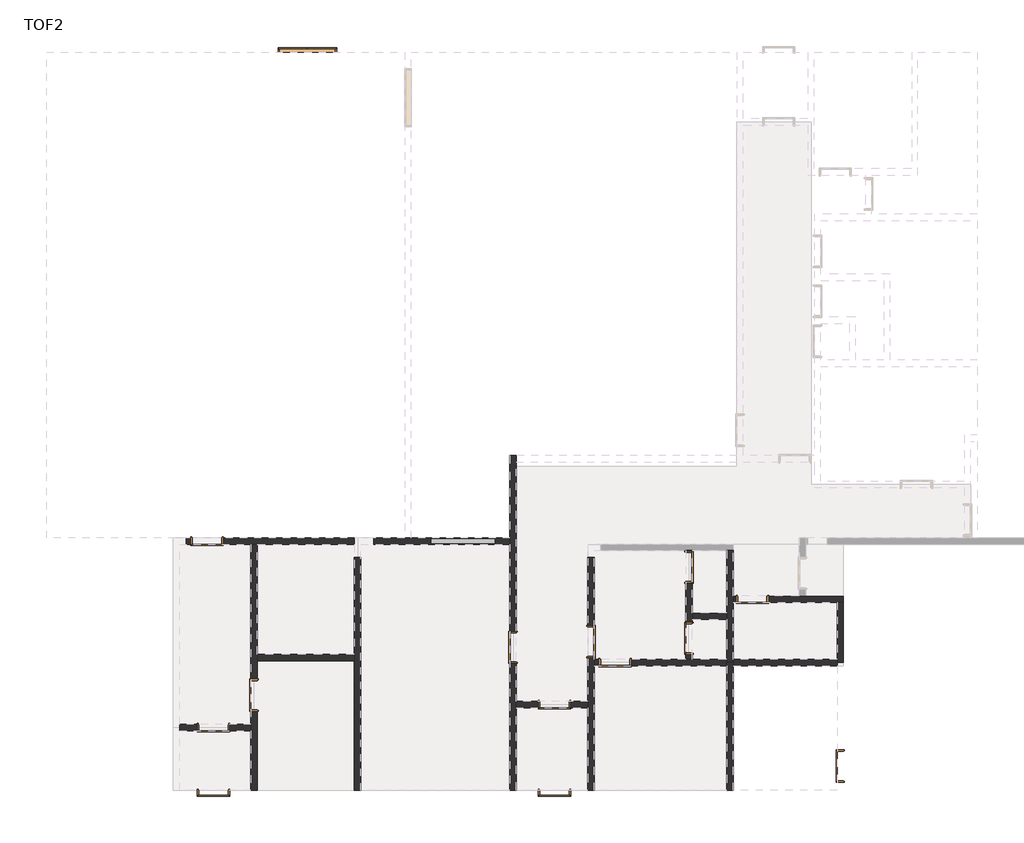
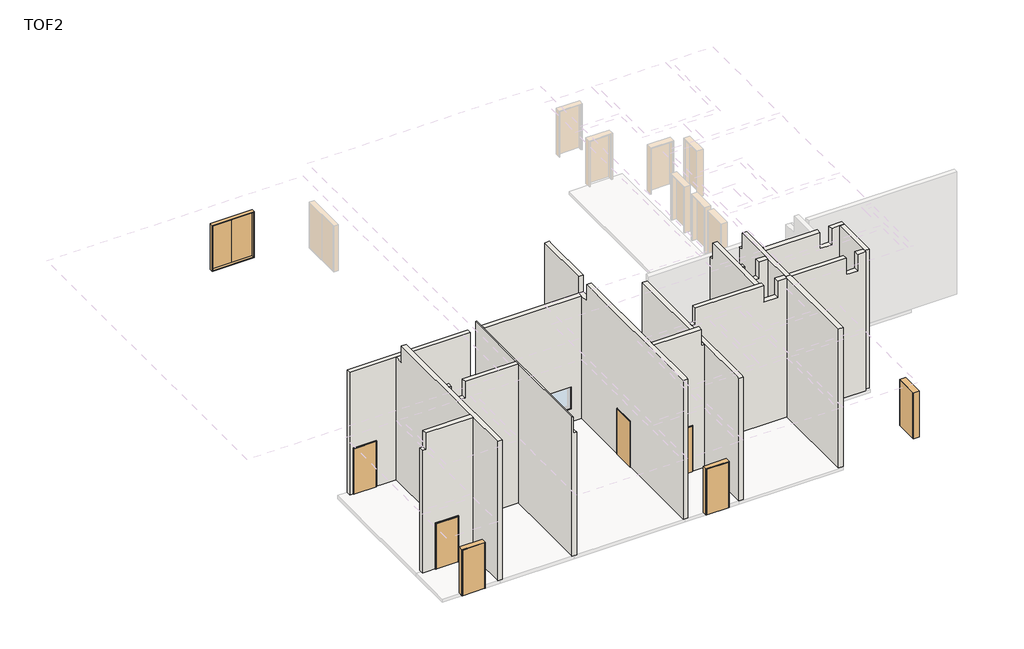
# One storey, part 1 of 2: 16 walls, 14 doors.
"""IFC4 building model written with IfcOpenShell, lengths in millimetres."""

import ifcopenshell
import ifcopenshell.guid

model = None  # the IFC model being written
_history = None  # IfcOwnerHistory: only IFC2X3 demands one
_inside = {}  # id of a spatial element -> (the spatial element, [elements in it])
_under = {}  # id of a project, library or spatial element -> (it, [spatial elements below it])
_declared = {}  # id of a project -> (the project, [libraries it declares])
_typed = {}  # id of a type object -> (the type object, [elements of that type])
_made_of = {}  # id of a material, layer set ... -> (it, [elements and type objects made of it])


def new_model(schema):
    """Start an empty IFC model of exactly this schema.

    Asked for "IFC4X3", IfcOpenShell would pick the latest addendum, in which some entities
    have other attributes; the version numbers below select the first issue.
    IFC2X3 requires an IfcOwnerHistory on every rooted entity: one is made here for all.
    """
    global model, _history
    if schema == "IFC4X3":
        model = ifcopenshell.file(schema_version=(4, 3, 0, 0))
    else:
        model = ifcopenshell.file(schema=schema)
    _inside.clear()
    _under.clear()
    _declared.clear()
    _typed.clear()
    _made_of.clear()
    _history = None
    if model.schema == "IFC2X3":
        org = make("IfcOrganization", Name="unknown")
        user = make(
            "IfcPersonAndOrganization",
            ThePerson=make("IfcPerson", FamilyName="unknown"),
            TheOrganization=org,
        )
        app = make(
            "IfcApplication",
            ApplicationDeveloper=org,
            Version="unknown",
            ApplicationFullName="unknown",
            ApplicationIdentifier="unknown",
        )
        _history = make(
            "IfcOwnerHistory",
            OwningUser=user,
            OwningApplication=app,
            ChangeAction="ADDED",
            CreationDate=0,
        )
    return model


def make(cls, **values):
    """One entity of the class cls with the attributes given. An attribute that is None is left unset."""
    return model.create_entity(
        cls, **{name: value for name, value in values.items() if value is not None}
    )


def rooted(cls, **values):
    """An entity with a GlobalId (a new one), such as an element, a storey or a relation."""
    return make(cls, GlobalId=ifcopenshell.guid.new(), OwnerHistory=_history, **values)


def si_unit(unit_type, name, prefix=None):
    """IfcSIUnit, for example si_unit("LENGTHUNIT", "METRE", prefix="MILLI")."""
    return make("IfcSIUnit", UnitType=unit_type, Prefix=prefix, Name=name)


def assignment(units):
    """IfcUnitAssignment: the units of a project."""
    return None if units is None else make("IfcUnitAssignment", Units=units)


def point(xyz):
    """IfcCartesianPoint."""
    return None if xyz is None else make("IfcCartesianPoint", Coordinates=xyz)


def direction(xyz):
    """IfcDirection."""
    return None if xyz is None else make("IfcDirection", DirectionRatios=xyz)


def frame(location, z_axis=None, x_axis=None):
    """IfcAxis2Placement3D, a coordinate frame: its origin and axes. An axis left out is left unset."""
    return make(
        "IfcAxis2Placement3D",
        Location=point(location),
        Axis=direction(z_axis),
        RefDirection=direction(x_axis),
    )


def origin():
    """The frame at (0, 0, 0) with its axes left unset."""
    return frame((0.0, 0.0, 0.0))


def origin_with_axes():
    """The frame at (0, 0, 0) with the z axis (0, 0, 1) and the x axis (1, 0, 0) written out."""
    return frame((0.0, 0.0, 0.0), z_axis=(0.0, 0.0, 1.0), x_axis=(1.0, 0.0, 0.0))


def place(relative_to, where):
    """IfcLocalPlacement: puts the frame where relative to a parent placement (None: the world)."""
    return make(
        "IfcLocalPlacement", PlacementRelTo=relative_to, RelativePlacement=where
    )


def context(
    kind, dimensions, precision=None, world=None, true_north=None, identifier=None
):
    """IfcGeometricRepresentationContext, for example the 3D "Model" context."""
    return make(
        "IfcGeometricRepresentationContext",
        ContextIdentifier=identifier,
        ContextType=kind,
        CoordinateSpaceDimension=dimensions,
        Precision=precision,
        WorldCoordinateSystem=world,
        TrueNorth=true_north,
    )


def project(units=None, contexts=None):
    """IfcProject with its units and contexts."""
    return rooted(
        "IfcProject",
        Name="project",
        RepresentationContexts=contexts,
        UnitsInContext=assignment(units),
    )


def spatial(cls, under=None, at=None, **own):
    """A site, building, storey or space (cls), placed at a placement, below another one or the project."""
    s = rooted(cls, ObjectPlacement=at, **own)
    if under is not None:
        _under.setdefault(under.id(), (under, []))[1].append(s)
    return s


def polyline(points):
    """IfcPolyline through the points."""
    return make("IfcPolyline", Points=[point(p) for p in points])


def outline(outer, holes=None, kind="AREA"):
    """IfcArbitraryClosedProfileDef: a profile drawn as a closed curve; with holes, ...WithVoids."""
    if holes is None:
        return make("IfcArbitraryClosedProfileDef", ProfileType=kind, OuterCurve=outer)
    return make(
        "IfcArbitraryProfileDefWithVoids",
        ProfileType=kind,
        OuterCurve=outer,
        InnerCurves=holes,
    )


def extrude(swept, where, along, depth):
    """IfcExtrudedAreaSolid: the profile swept, set in the frame where, extruded along a direction by depth."""
    return make(
        "IfcExtrudedAreaSolid",
        SweptArea=swept,
        Position=where,
        ExtrudedDirection=direction(along),
        Depth=depth,
    )


def faces_of(points, faces, orient=None, outer=None):
    """IfcFace entities. A face is a list of loops; a loop is a list of indices into points, from 0.

    orient and outer hold one flag for each loop. By default every Orientation is true, the
    first loop of a face is its IfcFaceOuterBound and the others are IfcFaceBound.
    """
    made = []
    for i, loops in enumerate(faces):
        bounds = []
        for j, loop in enumerate(loops):
            is_outer = j == 0 if outer is None else outer[i][j]
            bounds.append(
                make(
                    "IfcFaceOuterBound" if is_outer else "IfcFaceBound",
                    Bound=make("IfcPolyLoop", Polygon=[points[k] for k in loop]),
                    Orientation=True if orient is None else orient[i][j],
                )
            )
        made.append(make("IfcFace", Bounds=bounds))
    return made


def faceted_brep(points, faces, orient=None, outer=None, voids=None):
    """IfcFacetedBrep: a solid bounded by flat faces; with voids (closed shells), ...WithVoids."""
    shared = [point(p) for p in points]
    hull = make("IfcClosedShell", CfsFaces=faces_of(shared, faces, orient, outer))
    if voids is None:
        return make("IfcFacetedBrep", Outer=hull)
    return make(
        "IfcFacetedBrepWithVoids",
        Outer=hull,
        Voids=[
            make(cls, CfsFaces=faces_of(shared, fs, o, b)) for cls, fs, o, b in voids
        ],
    )


def shape(context_of_items, identifier, shape_type, items):
    """IfcShapeRepresentation: the items that make up one representation, for example the "Body"."""
    return make(
        "IfcShapeRepresentation",
        ContextOfItems=context_of_items,
        RepresentationIdentifier=identifier,
        RepresentationType=shape_type,
        Items=items,
    )


def source(mapping_origin, context_of_items, identifier, shape_type, items):
    """IfcRepresentationMap: a shape defined once, which mapped items show again and again."""
    return make(
        "IfcRepresentationMap",
        MappingOrigin=mapping_origin,
        MappedRepresentation=shape(context_of_items, identifier, shape_type, items),
    )


def transform(
    local_origin,
    x_axis=None,
    y_axis=None,
    z_axis=None,
    scale=None,
    scale2=None,
    scale3=None,
    uniform=True,
):
    """IfcCartesianTransformationOperator3D, or its non-uniform kind. x_axis, y_axis, z_axis: its Axis1, 2, 3."""
    if uniform:
        return make(
            "IfcCartesianTransformationOperator3D",
            Axis1=direction(x_axis),
            Axis2=direction(y_axis),
            LocalOrigin=point(local_origin),
            Scale=scale,
            Axis3=direction(z_axis),
        )
    return make(
        "IfcCartesianTransformationOperator3DnonUniform",
        Axis1=direction(x_axis),
        Axis2=direction(y_axis),
        LocalOrigin=point(local_origin),
        Scale=scale,
        Axis3=direction(z_axis),
        Scale2=scale2,
        Scale3=scale3,
    )


def mapped(mapping_source, mapping_target):
    """IfcMappedItem: shows the shape of a source again, moved by a transform."""
    return make(
        "IfcMappedItem", MappingSource=mapping_source, MappingTarget=mapping_target
    )


def made_of(thing, what):
    """Note that an element or type object is made of a material, layer set ...; save() writes the relation."""
    if what is not None:
        _made_of.setdefault(what.id(), (what, []))[1].append(thing)
    return thing


def element(
    cls,
    number,
    at=None,
    inside=None,
    cuts=None,
    type_object=None,
    material=None,
    context=None,
    identifier="Body",
    shape_type=None,
    held_by="IfcProductDefinitionShape",
    body=None,
    shapes=None,
    **own,
):
    """One element of the class cls, such as IfcWall. Its Tag is "e" and its number.

    at: its placement. inside: the storey or other place that contains it. cuts: it is an
    opening in that element (IfcRelVoidsElement). A single representation is given by context,
    identifier, shape_type and body (its items); several are given by shapes. held_by: the class
    of the entity that holds the representations. save() writes the other relations.
    """
    e = rooted(cls, Tag="e%d" % number, ObjectPlacement=at, **own)
    if body is not None:
        shapes = [shape(context, identifier, shape_type, body)]
    if shapes is not None:
        e.Representation = make(held_by, Representations=shapes)
    if inside is not None:
        _inside.setdefault(inside.id(), (inside, []))[1].append(e)
    if cuts is not None:
        rooted(
            "IfcRelVoidsElement", RelatingBuildingElement=cuts, RelatedOpeningElement=e
        )
    if type_object is not None:
        _typed.setdefault(type_object.id(), (type_object, []))[1].append(e)
    return made_of(e, material)


def aggregate(whole, parts):
    """IfcRelAggregates: a whole, such as a stair, and the parts it consists of."""
    return rooted("IfcRelAggregates", RelatingObject=whole, RelatedObjects=parts)


def save(model, path):
    """Write the relations noted so far, then the file.

    IfcRelAggregates (storeys below a building ...), IfcRelContainedInSpatialStructure (elements
    in a storey), IfcRelDefinesByType, IfcRelAssociatesMaterial and IfcRelDeclares: one each for
    every whole, place, type object, material and project.
    """
    for whole, parts in _under.values():
        aggregate(whole, parts)
    for where, things in _inside.values():
        rooted(
            "IfcRelContainedInSpatialStructure",
            RelatedElements=things,
            RelatingStructure=where,
        )
    for kind, things in _typed.values():
        rooted("IfcRelDefinesByType", RelatedObjects=things, RelatingType=kind)
    for what, things in _made_of.values():
        rooted("IfcRelAssociatesMaterial", RelatedObjects=things, RelatingMaterial=what)
    for by, libraries in _declared.values():
        rooted("IfcRelDeclares", RelatingContext=by, RelatedDefinitions=libraries)
    model.write(path)


def double_door_steel_580823b0(model_context):
    return source(origin(), model_context, "Body", "SolidModel", [
        extrude(outline(polyline([(880.0, 35.0), (0.0, 35.0), (0.0, 75.0), (880.0, 75.0), (880.0, 35.0)])), frame((0.0, 0.0, 20.0), z_axis=(0.0, 0.0, 1.0), x_axis=(1.0, 0.0, 0.0)), (0.0, 0.0, 1.0), 2060.0),
        extrude(outline(polyline([(0.0, 35.0), (-880.0, 35.0), (-880.0, 75.0), (0.0, 75.0), (0.0, 35.0)])), frame((0.0, 0.0, 20.0), z_axis=(0.0, 0.0, 1.0), x_axis=(1.0, 0.0, 0.0)), (0.0, 0.0, 1.0), 2060.0),
        faceted_brep([(900.0, -75.0, 2100.0), (900.0, 75.0, 2100.0), (-900.0, 75.0, 2100.0), (-900.0, -75.0, 2100.0), (865.0, 35.0, 2065.0), (865.0, -75.0, 2065.0), (-865.0, -75.0, 2065.0), (-865.0, 35.0, 2065.0), (880.0, 75.0, 2080.0), (880.0, 35.0, 2080.0), (-880.0, 35.0, 2080.0), (-880.0, 75.0, 2080.0), (-900.0, 75.0, 0.0), (-900.0, -75.0, 0.0), (-865.0, -75.0, 35.0), (-865.0, 35.0, 35.0), (-880.0, 35.0, 20.0), (-880.0, 75.0, 20.0), (900.0, 75.0, 0.0), (880.0, 75.0, 20.0), (900.0, -75.0, 0.0), (865.0, -75.0, 35.0), (865.0, 35.0, 35.0), (880.0, 35.0, 20.0)], [[[0, 1, 2, 3]], [[4, 5, 6, 7]], [[8, 9, 10, 11]], [[3, 2, 12, 13]], [[7, 6, 14, 15]], [[11, 10, 16, 17]], [[18, 12, 2, 1], [8, 11, 17, 19]], [[13, 12, 18, 20]], [[0, 3, 13, 20], [21, 14, 6, 5]], [[15, 14, 21, 22]], [[23, 16, 10, 9], [4, 7, 15, 22]], [[17, 16, 23, 19]], [[20, 18, 1, 0]], [[22, 21, 5, 4]], [[19, 23, 9, 8]]]),
    ])


def single_door_steel_02f153ad(model_context):
    return source(origin(), model_context, "Body", "SolidModel", [
        extrude(outline(polyline([(470.0, -130.0), (-470.0, -130.0), (-470.0, -95.0), (470.0, -95.0), (470.0, -130.0)])), origin_with_axes(), (0.0, 0.0, 1.0), 2070.0),
        faceted_brep([(470.0, -130.0, 0.0), (470.0, -95.0, 0.0), (450.0, -95.0, 0.0), (450.0, 95.0, 0.0), (470.0, 95.0, 0.0), (470.0, 130.0, 0.0), (500.0, 130.0, 0.0), (500.0, -130.0, 0.0), (500.0, -130.0, 2100.0), (-500.0, -130.0, 2100.0), (-500.0, -130.0, 0.0), (-470.0, -130.0, 0.0), (-470.0, -130.0, 2070.0), (470.0, -130.0, 2070.0), (500.0, 130.0, 2100.0), (470.0, 130.0, 2070.0), (-470.0, 130.0, 2070.0), (-470.0, 130.0, 0.0), (-500.0, 130.0, 0.0), (-500.0, 130.0, 2100.0), (470.0, 95.0, 2070.0), (450.0, 95.0, 2050.0), (-450.0, 95.0, 2050.0), (-450.0, 95.0, 0.0), (-470.0, 95.0, 0.0), (-470.0, 95.0, 2070.0), (450.0, -95.0, 2050.0), (470.0, -95.0, 2070.0), (-470.0, -95.0, 2070.0), (-470.0, -95.0, 0.0), (-450.0, -95.0, 0.0), (-450.0, -95.0, 2050.0)], [[[0, 1, 2, 3, 4, 5, 6, 7]], [[7, 8, 9, 10, 11, 12, 13, 0]], [[6, 14, 8, 7]], [[5, 15, 16, 17, 18, 19, 14, 6]], [[4, 20, 15, 5]], [[3, 21, 22, 23, 24, 25, 20, 4]], [[2, 26, 21, 3]], [[1, 27, 28, 29, 30, 31, 26, 2]], [[0, 13, 27, 1]], [[12, 11, 29, 28]], [[11, 10, 18, 17, 24, 23, 30, 29]], [[19, 18, 10, 9]], [[25, 24, 17, 16]], [[31, 30, 23, 22]], [[14, 19, 9, 8]], [[20, 25, 16, 15]], [[26, 31, 22, 21]], [[13, 12, 28, 27]]]),
    ])


def single_door_steel_4a6c7de9(model_context):
    return source(origin(), model_context, "Body", "SolidModel", [
        extrude(outline(polyline([(470.0, 130.0), (470.0, 95.0), (-470.0, 95.0), (-470.0, 130.0), (470.0, 130.0)])), origin_with_axes(), (0.0, 0.0, 1.0), 2070.0),
        faceted_brep([(470.0, 130.0, 0.0), (500.0, 130.0, 0.0), (500.0, -130.0, 0.0), (470.0, -130.0, 0.0), (470.0, -95.0, 0.0), (450.0, -95.0, 0.0), (450.0, 95.0, 0.0), (470.0, 95.0, 0.0), (470.0, 130.0, 2070.0), (-470.0, 130.0, 2070.0), (-470.0, 130.0, 0.0), (-500.0, 130.0, 0.0), (-500.0, 130.0, 2100.0), (500.0, 130.0, 2100.0), (500.0, -130.0, 2100.0), (-500.0, -130.0, 2100.0), (-500.0, -130.0, 0.0), (-470.0, -130.0, 0.0), (-470.0, -130.0, 2070.0), (470.0, -130.0, 2070.0), (470.0, -95.0, 2070.0), (-470.0, -95.0, 2070.0), (-470.0, -95.0, 0.0), (-450.0, -95.0, 0.0), (-450.0, -95.0, 2050.0), (450.0, -95.0, 2050.0), (450.0, 95.0, 2050.0), (-450.0, 95.0, 2050.0), (-450.0, 95.0, 0.0), (-470.0, 95.0, 0.0), (-470.0, 95.0, 2070.0), (470.0, 95.0, 2070.0)], [[[0, 1, 2, 3, 4, 5, 6, 7]], [[1, 0, 8, 9, 10, 11, 12, 13]], [[2, 1, 13, 14]], [[3, 2, 14, 15, 16, 17, 18, 19]], [[4, 3, 19, 20]], [[5, 4, 20, 21, 22, 23, 24, 25]], [[6, 5, 25, 26]], [[7, 6, 26, 27, 28, 29, 30, 31]], [[0, 7, 31, 8]], [[9, 30, 29, 10]], [[10, 29, 28, 23, 22, 17, 16, 11]], [[15, 12, 11, 16]], [[21, 18, 17, 22]], [[27, 24, 23, 28]], [[14, 13, 12, 15]], [[20, 19, 18, 21]], [[26, 25, 24, 27]], [[8, 31, 30, 9]]]),
    ])


def single_door_steel_8d57826b(model_context):
    return source(origin(), model_context, "Body", "SolidModel", [
        extrude(outline(polyline([(470.0, -105.0), (-470.0, -105.0), (-470.0, -70.0), (470.0, -70.0), (470.0, -105.0)])), origin_with_axes(), (0.0, 0.0, 1.0), 2070.0),
        faceted_brep([(470.0, -105.0, 0.0), (470.0, -70.0, 0.0), (450.0, -70.0, 0.0), (450.0, 70.0, 0.0), (470.0, 70.0, 0.0), (470.0, 105.0, 0.0), (500.0, 105.0, 0.0), (500.0, -105.0, 0.0), (500.0, -105.0, 2100.0), (-500.0, -105.0, 2100.0), (-500.0, -105.0, 0.0), (-470.0, -105.0, 0.0), (-470.0, -105.0, 2070.0), (470.0, -105.0, 2070.0), (500.0, 105.0, 2100.0), (470.0, 105.0, 2070.0), (-470.0, 105.0, 2070.0), (-470.0, 105.0, 0.0), (-500.0, 105.0, 0.0), (-500.0, 105.0, 2100.0), (470.0, 70.0, 2070.0), (450.0, 70.0, 2050.0), (-450.0, 70.0, 2050.0), (-450.0, 70.0, 0.0), (-470.0, 70.0, 0.0), (-470.0, 70.0, 2070.0), (450.0, -70.0, 2050.0), (470.0, -70.0, 2070.0), (-470.0, -70.0, 2070.0), (-470.0, -70.0, 0.0), (-450.0, -70.0, 0.0), (-450.0, -70.0, 2050.0)], [[[0, 1, 2, 3, 4, 5, 6, 7]], [[7, 8, 9, 10, 11, 12, 13, 0]], [[6, 14, 8, 7]], [[5, 15, 16, 17, 18, 19, 14, 6]], [[4, 20, 15, 5]], [[3, 21, 22, 23, 24, 25, 20, 4]], [[2, 26, 21, 3]], [[1, 27, 28, 29, 30, 31, 26, 2]], [[0, 13, 27, 1]], [[12, 11, 29, 28]], [[11, 10, 18, 17, 24, 23, 30, 29]], [[19, 18, 10, 9]], [[25, 24, 17, 16]], [[31, 30, 23, 22]], [[14, 19, 9, 8]], [[20, 25, 16, 15]], [[26, 31, 22, 21]], [[13, 12, 28, 27]]]),
    ])


def single_door_steel_6218e75e(model_context):
    return source(origin(), model_context, "Body", "SolidModel", [
        extrude(outline(polyline([(470.0, 105.0), (470.0, 70.0), (-470.0, 70.0), (-470.0, 105.0), (470.0, 105.0)])), origin_with_axes(), (0.0, 0.0, 1.0), 2070.0),
        faceted_brep([(470.0, 105.0, 0.0), (500.0, 105.0, 0.0), (500.0, -105.0, 0.0), (470.0, -105.0, 0.0), (470.0, -70.0, 0.0), (450.0, -70.0, 0.0), (450.0, 70.0, 0.0), (470.0, 70.0, 0.0), (470.0, 105.0, 2070.0), (-470.0, 105.0, 2070.0), (-470.0, 105.0, 0.0), (-500.0, 105.0, 0.0), (-500.0, 105.0, 2100.0), (500.0, 105.0, 2100.0), (500.0, -105.0, 2100.0), (-500.0, -105.0, 2100.0), (-500.0, -105.0, 0.0), (-470.0, -105.0, 0.0), (-470.0, -105.0, 2070.0), (470.0, -105.0, 2070.0), (470.0, -70.0, 2070.0), (-470.0, -70.0, 2070.0), (-470.0, -70.0, 0.0), (-450.0, -70.0, 0.0), (-450.0, -70.0, 2050.0), (450.0, -70.0, 2050.0), (450.0, 70.0, 2050.0), (-450.0, 70.0, 2050.0), (-450.0, 70.0, 0.0), (-470.0, 70.0, 0.0), (-470.0, 70.0, 2070.0), (470.0, 70.0, 2070.0)], [[[0, 1, 2, 3, 4, 5, 6, 7]], [[1, 0, 8, 9, 10, 11, 12, 13]], [[2, 1, 13, 14]], [[3, 2, 14, 15, 16, 17, 18, 19]], [[4, 3, 19, 20]], [[5, 4, 20, 21, 22, 23, 24, 25]], [[6, 5, 25, 26]], [[7, 6, 26, 27, 28, 29, 30, 31]], [[0, 7, 31, 8]], [[9, 30, 29, 10]], [[10, 29, 28, 23, 22, 17, 16, 11]], [[15, 12, 11, 16]], [[21, 18, 17, 22]], [[27, 24, 23, 28]], [[14, 13, 12, 15]], [[20, 19, 18, 21]], [[26, 25, 24, 27]], [[8, 31, 30, 9]]]),
    ])


model = new_model("IFC4")

# Units and contexts
model_context = context("Model", 3, world=origin())
ifc_project = project(units=[si_unit("LENGTHUNIT", "METRE", prefix="MILLI")], contexts=[model_context])

# Site, building, storey
site = spatial("IfcSite", under=ifc_project)
building = spatial("IfcBuilding", under=site)
storey = spatial("IfcBuildingStorey", under=building, Name="TOF2", Elevation=1149.9618634)

# Doors
placement = place(None, origin())
double_door_steel_shape = double_door_steel_580823b0(model_context)
element("IfcDoor", 1, ObjectType="Double Door_Steel : H_DR_AR_B12_Double Door_Steel_W2000xH2100", at=placement, inside=storey, context=model_context, shape_type="MappedRepresentation", body=[
    mapped(double_door_steel_shape, transform((30250.0, 23674.5208589, 1149.9618634), x_axis=(1.0, 0.0, 0.0), y_axis=(0.0, 1.0, 0.0), z_axis=(0.0, 0.0, 1.0))),
])
single_door_steel_shape = single_door_steel_02f153ad(model_context)
element("IfcDoor", 2, ObjectType="Single Door_Steel : H_DR_AR_B12_Single Door_Steel_W1000xH2100", at=placement, inside=storey, context=model_context, shape_type="MappedRepresentation", body=[
    mapped(single_door_steel_shape, transform((27150.0, 8499.5208589, 1149.9618634), x_axis=(1.0, 0.0, 0.0), y_axis=(0.0, 1.0, 0.0), z_axis=(0.0, 0.0, 1.0))),
])
element("IfcDoor", 3, ObjectType="Single Door_Steel : H_DR_AR_B12_Single Door_Steel_W1000xH2100", at=placement, inside=storey, context=model_context, shape_type="MappedRepresentation", body=[
    mapped(single_door_steel_shape, transform((28600.0, 3737.0208589, 1149.9618634), x_axis=(0.0, -1.0, 0.0), y_axis=(1.0, 0.0, 0.0), z_axis=(0.0, 0.0, 1.0))),
])
element("IfcDoor", 4, ObjectType="Single Door_Steel : H_DR_AR_B12_Single Door_Steel_W1000xH2100", at=placement, inside=storey, context=model_context, shape_type="MappedRepresentation", body=[
    mapped(single_door_steel_shape, transform((27350.0, 2737.0208589, 1149.9618634), x_axis=(1.0, 0.0, 0.0), y_axis=(0.0, 1.0, 0.0), z_axis=(0.0, 0.0, 1.0))),
])
element("IfcDoor", 5, ObjectType="Single Door_Steel : H_DR_AR_B12_Single Door_Steel_W1000xH2100", at=placement, inside=storey, context=model_context, shape_type="MappedRepresentation", body=[
    mapped(single_door_steel_shape, transform((43985.0, 6699.5208589, 1149.9618634), x_axis=(1.0, 0.0, 0.0), y_axis=(0.0, 1.0, 0.0), z_axis=(0.0, 0.0, 1.0))),
])
single_door_steel_2_shape = single_door_steel_4a6c7de9(model_context)
element("IfcDoor", 6, ObjectType="Single Door_Steel : H_DR_AR_B12_Single Door_Steel_W1000xH2100", at=placement, inside=storey, context=model_context, shape_type="MappedRepresentation", body=[
    mapped(single_door_steel_2_shape, transform((36600.0, 5218.8249516, 1149.9618634), x_axis=(0.0, 1.0, 0.0), y_axis=(-1.0, 0.0, 0.0), z_axis=(0.0, 0.0, 1.0))),
])
element("IfcDoor", 7, ObjectType="Single Door_Steel : H_DR_AR_B12_Single Door_Steel_W1000xH2100", at=placement, inside=storey, context=model_context, shape_type="MappedRepresentation", body=[
    mapped(single_door_steel_2_shape, transform((37875.0, 3443.8249516, 1149.9618634), x_axis=(-1.0, 0.0, 0.0), y_axis=(0.0, -1.0, 0.0), z_axis=(0.0, 0.0, 1.0))),
])
element("IfcDoor", 8, ObjectType="Single Door_Steel : H_DR_AR_B12_Single Door_Steel_W1000xH2100", at=placement, inside=storey, context=model_context, shape_type="MappedRepresentation", body=[
    mapped(single_door_steel_2_shape, transform((46700.0, 1549.5208589, 1149.9618634), x_axis=(0.0, 1.0, 0.0), y_axis=(-1.0, 0.0, 0.0), z_axis=(0.0, 0.0, 1.0))),
])
element("IfcDoor", 9, ObjectType="Single Door_Steel : H_DR_AR_B12_Single Door_Steel_W1000xH2100", at=placement, inside=storey, context=model_context, shape_type="MappedRepresentation", body=[
    mapped(single_door_steel_2_shape, transform((39000.0, 5393.8249516, 1149.9618634), x_axis=(0.0, -1.0, 0.0), y_axis=(1.0, 0.0, 0.0), z_axis=(0.0, 0.0, 1.0))),
])
element("IfcDoor", 10, ObjectType="Single Door_Steel : H_DR_AR_B12_Single Door_Steel_W1000xH2100", at=placement, inside=storey, context=model_context, shape_type="MappedRepresentation", body=[
    mapped(single_door_steel_2_shape, transform((39750.0, 4749.5208589, 1149.9618634), x_axis=(-1.0, 0.0, 0.0), y_axis=(0.0, -1.0, 0.0), z_axis=(0.0, 0.0, 1.0))),
])
element("IfcDoor", 11, ObjectType="Single Door_Steel : H_DR_AR_B12_Single Door_Steel_W1000xH2100", at=placement, inside=storey, context=model_context, shape_type="MappedRepresentation", body=[
    mapped(single_door_steel_2_shape, transform((42025.0, 7699.5208589, 1149.9618634), x_axis=(0.0, -1.0, 0.0), y_axis=(1.0, 0.0, 0.0), z_axis=(0.0, 0.0, 1.0))),
])
element("IfcDoor", 12, ObjectType="Single Door_Steel : H_DR_AR_B12_Single Door_Steel_W1000xH2100", at=placement, inside=storey, context=model_context, shape_type="MappedRepresentation", body=[
    mapped(single_door_steel_2_shape, transform((42025.0, 5496.6729053, 1149.9618634), x_axis=(0.0, 1.0, 0.0), y_axis=(-1.0, 0.0, 0.0), z_axis=(0.0, 0.0, 1.0))),
])
single_door_steel_3_shape = single_door_steel_8d57826b(model_context)
element("IfcDoor", 13, ObjectType="Single Door_Steel : H_DR_AR_B12_Single Door_Steel_W1000xH2100", at=placement, inside=storey, context=model_context, shape_type="MappedRepresentation", body=[
    mapped(single_door_steel_3_shape, transform((27350.0, 724.5208589, 1149.9618634), x_axis=(1.0, 0.0, 0.0), y_axis=(0.0, 1.0, 0.0), z_axis=(0.0, 0.0, 1.0))),
])
single_door_steel_4_shape = single_door_steel_6218e75e(model_context)
element("IfcDoor", 14, ObjectType="Single Door_Steel : H_DR_AR_B12_Single Door_Steel_W1000xH2100", at=placement, inside=storey, context=model_context, shape_type="MappedRepresentation", body=[
    mapped(single_door_steel_4_shape, transform((37875.0, 724.5208589, 1149.9618634), x_axis=(-1.0, 0.0, 0.0), y_axis=(0.0, -1.0, 0.0), z_axis=(0.0, 0.0, 1.0))),
])

# Walls
element("IfcWall", 15, ObjectType="H_WA_AR_B02_Int Wall_Block T200", at=placement, inside=storey, context=model_context, shape_type="Brep", body=[
    faceted_brep([(26500.0, 8599.5208589, 1149.9618634), (26500.0, 8599.5208589, 6749.9618634), (31700.0, 8599.5208589, 6749.9618634), (31700.0, 8599.5208589, 1149.9618634), (28600.0, 8599.5208589, 1149.9618634), (27650.0, 8599.5208589, 1149.9618634), (27650.0, 8599.5208589, 3249.9618634), (26650.0, 8599.5208589, 3249.9618634), (26650.0, 8599.5208589, 1149.9618634), (26500.0, 8399.5208589, 6749.9618634), (26500.0, 8399.5208589, 1149.9618634), (26650.0, 8399.5208589, 1149.9618634), (26650.0, 8399.5208589, 3249.9618634), (27650.0, 8399.5208589, 3249.9618634), (27650.0, 8399.5208589, 1149.9618634), (28500.0, 8399.5208589, 1149.9618634), (28700.0, 8399.5208589, 1149.9618634), (31700.0, 8399.5208589, 1149.9618634), (31700.0, 8399.5208589, 6749.9618634), (28700.0, 8399.5208589, 6749.9618634), (28500.0, 8399.5208589, 6749.9618634)], [[[0, 1, 2, 3, 4, 5, 6, 7, 8]], [[9, 10, 11, 12, 13, 14, 15, 16, 17, 18, 19, 20]], [[10, 0, 8, 11]], [[3, 17, 16, 15, 14, 5, 4]], [[0, 10, 9, 1]], [[17, 3, 2, 18]], [[2, 1, 9, 20, 19, 18]], [[13, 6, 5, 14]], [[6, 13, 12, 7]], [[7, 12, 11, 8]]]),
    faceted_brep([(36500.0, 8599.5208589, 1149.9618634), (32300.0, 8599.5208589, 1149.9618634), (32300.0, 8599.5208589, 6749.9618634), (36500.0, 8599.5208589, 6749.9618634), (36050.0, 8599.5208589, 1749.9618634), (36050.0, 8599.5208589, 2749.9618634), (34050.0, 8599.5208589, 2749.9618634), (34050.0, 8599.5208589, 1749.9618634), (32300.0, 8399.5208589, 1149.9618634), (36500.0, 8399.5208589, 1149.9618634), (36500.0, 8399.5208589, 6749.9618634), (32300.0, 8399.5208589, 6749.9618634), (36050.0, 8399.5208589, 2749.9618634), (36050.0, 8399.5208589, 1749.9618634), (34050.0, 8399.5208589, 1749.9618634), (34050.0, 8399.5208589, 2749.9618634)], [[[0, 1, 2, 3], [4, 5, 6, 7]], [[8, 9, 10, 11], [12, 13, 14, 15]], [[0, 9, 8, 1]], [[9, 0, 3, 10]], [[5, 4, 13, 12]], [[6, 5, 12, 15]], [[7, 6, 15, 14]], [[4, 7, 14, 13]], [[1, 8, 11, 2]], [[3, 2, 11, 10]]]),
])
element("IfcWall", 16, ObjectType="H_WA_AR_B02_Int Wall_Block T200", at=placement, inside=storey, context=model_context, shape_type="Brep", body=[
    faceted_brep([(31700.0, 7999.5208589, 1149.9618634), (31700.0, 4999.0208589, 1149.9618634), (31700.0, 4799.0208589, 1149.9618634), (31700.0, 925.5208589, 1149.9618634), (31700.0, 799.5208589, 1149.9618634), (31700.0, 799.5208589, 7499.9618634), (31700.0, 925.5208589, 7499.9618634), (31700.0, 4799.0208589, 7499.9618634), (31700.0, 4999.0208589, 7499.9618634), (31700.0, 7999.5208589, 7499.9618634), (31900.0, 799.5208589, 1149.9618634), (31900.0, 925.5208589, 1149.9618634), (31900.0, 7999.5208589, 1149.9618634), (31900.0, 7999.5208589, 6749.9618634), (31900.0, 925.5208589, 6749.9618634), (31900.0, 799.5208589, 6749.9618634), (31750.0, 799.5208589, 6749.9618634), (31750.0, 799.5208589, 7499.9618634), (31750.0, 7999.5208589, 7499.9618634), (31750.0, 7999.5208589, 6749.9618634)], [[[0, 1, 2, 3, 4, 5, 6, 7, 8, 9]], [[10, 11, 12, 13, 14, 15]], [[10, 4, 3, 2, 1, 0, 12, 11]], [[4, 10, 15, 16, 17, 5]], [[12, 0, 9, 18, 19, 13]], [[19, 16, 15, 14, 13]], [[16, 19, 18, 17]], [[9, 8, 7, 6, 5, 17, 18]]]),
])
element("IfcWall", 17, ObjectType="H_WA_AR_B02_Int Wall_Block T200", at=placement, inside=storey, context=model_context, shape_type="Brep", body=[
    faceted_brep([(36500.0, 11149.5208589, 1149.9618634), (36500.0, 8599.5208589, 1149.9618634), (36500.0, 8399.5208589, 1149.9618634), (36500.0, 5718.8249516, 1149.9618634), (36500.0, 5718.8249516, 3249.9618634), (36500.0, 4718.8249516, 3249.9618634), (36500.0, 4718.8249516, 1149.9618634), (36500.0, 925.5208589, 1149.9618634), (36500.0, 799.5208589, 1149.9618634), (36500.0, 799.5208589, 7499.9618634), (36500.0, 925.5208589, 7499.9618634), (36500.0, 7999.5208589, 7499.9618634), (36500.0, 7999.5208589, 6749.9618634), (36500.0, 8399.5208589, 6749.9618634), (36500.0, 8599.5208589, 6749.9618634), (36500.0, 8599.5208589, 7499.9618634), (36500.0, 11149.5208589, 7499.9618634), (36700.0, 5718.8249516, 1149.9618634), (36700.0, 11149.5208589, 1149.9618634), (36700.0, 11149.5208589, 7499.9618634), (36700.0, 10949.5208589, 7499.9618634), (36700.0, 8599.5208589, 7499.9618634), (36700.0, 8599.5208589, 6749.9618634), (36700.0, 7999.5208589, 6749.9618634), (36700.0, 7999.5208589, 7499.9618634), (36700.0, 3543.8249516, 7499.9618634), (36700.0, 3343.8249516, 7499.9618634), (36700.0, 925.5208589, 7499.9618634), (36700.0, 799.5208589, 7499.9618634), (36700.0, 799.5208589, 1149.9618634), (36700.0, 925.5208589, 1149.9618634), (36700.0, 3343.8249516, 1149.9618634), (36700.0, 3543.8249516, 1149.9618634), (36700.0, 4718.8249516, 1149.9618634), (36700.0, 4718.8249516, 3249.9618634), (36700.0, 5718.8249516, 3249.9618634)], [[[0, 1, 2, 3, 4, 5, 6, 7, 8, 9, 10, 11, 12, 13, 14, 15, 16]], [[17, 18, 19, 20, 21, 22, 23, 24, 25, 26, 27, 28, 29, 30, 31, 32, 33, 34, 35]], [[0, 18, 17, 3, 2, 1]], [[29, 8, 7, 6, 33, 32, 31, 30]], [[8, 29, 28, 9]], [[18, 0, 16, 19]], [[35, 4, 3, 17]], [[4, 35, 34, 5]], [[5, 34, 33, 6]], [[23, 12, 11, 24]], [[12, 23, 22, 14, 13]], [[14, 22, 21, 15]], [[16, 15, 21, 20, 19]], [[11, 10, 9, 28, 27, 26, 25, 24]]]),
])
element("IfcWall", 18, ObjectType="H_WA_AR_B02_Int Wall_Block T200", at=placement, inside=storey, context=model_context, shape_type="Brep", body=[
    faceted_brep([(39100.0, 799.5208589, 1149.9618634), (39100.0, 925.5208589, 1149.9618634), (39100.0, 4649.5208589, 1149.9618634), (39100.0, 4849.5208589, 1149.9618634), (39100.0, 4893.8249516, 1149.9618634), (39100.0, 4893.8249516, 3249.9618634), (39100.0, 5893.8249516, 3249.9618634), (39100.0, 5893.8249516, 1149.9618634), (39100.0, 7999.5208589, 1149.9618634), (39100.0, 7999.5208589, 6749.9618634), (39100.0, 4849.5208589, 6749.9618634), (39100.0, 4649.5208589, 6749.9618634), (39100.0, 925.5208589, 6749.9618634), (39100.0, 799.5208589, 6749.9618634), (38900.0, 4893.8249516, 1149.9618634), (38900.0, 3543.8249516, 1149.9618634), (38900.0, 3343.8249516, 1149.9618634), (38900.0, 925.5208589, 1149.9618634), (38900.0, 799.5208589, 1149.9618634), (38900.0, 799.5208589, 6749.9618634), (38900.0, 925.5208589, 6749.9618634), (38900.0, 3343.8249516, 6749.9618634), (38900.0, 3543.8249516, 6749.9618634), (38900.0, 7999.5208589, 6749.9618634), (38900.0, 7999.5208589, 1149.9618634), (38900.0, 5893.8249516, 1149.9618634), (38900.0, 5893.8249516, 3249.9618634), (38900.0, 4893.8249516, 3249.9618634)], [[[0, 1, 2, 3, 4, 5, 6, 7, 8, 9, 10, 11, 12, 13]], [[14, 15, 16, 17, 18, 19, 20, 21, 22, 23, 24, 25, 26, 27]], [[7, 25, 24, 8]], [[0, 18, 17, 16, 15, 14, 4, 3, 2, 1]], [[18, 0, 13, 19]], [[27, 5, 4, 14]], [[5, 27, 26, 6]], [[6, 26, 25, 7]], [[8, 24, 23, 9]], [[13, 12, 11, 10, 9, 23, 22, 21, 20, 19]]]),
])
element("IfcWall", 19, ObjectType="H_WA_AR_B02_Int Wall_Block T200", at=placement, inside=storey, context=model_context, shape_type="Brep", body=[
    faceted_brep([(43400.0, 799.5208589, 1149.9618634), (43400.0, 925.5208589, 1149.9618634), (43400.0, 4649.5208589, 1149.9618634), (43400.0, 4749.5208589, 1149.9618634), (43400.0, 4749.5208589, 7499.9618634), (43400.0, 4649.5208589, 7499.9618634), (43400.0, 925.5208589, 7499.9618634), (43400.0, 799.5208589, 7499.9618634), (43200.0, 4749.5208589, 1149.9618634), (43200.0, 4649.5208589, 1149.9618634), (43200.0, 925.5208589, 1149.9618634), (43200.0, 799.5208589, 1149.9618634), (43200.0, 799.5208589, 7499.9618634), (43200.0, 925.5208589, 7499.9618634), (43200.0, 4649.5208589, 7499.9618634), (43200.0, 4749.5208589, 7499.9618634)], [[[0, 1, 2, 3, 4, 5, 6, 7]], [[8, 9, 10, 11, 12, 13, 14, 15]], [[3, 2, 1, 0, 11, 10, 9, 8]], [[3, 8, 15, 4]], [[11, 0, 7, 12]], [[7, 6, 5, 4, 15, 14, 13, 12]]]),
])
element("IfcWall", 20, ObjectType="H_WA_AR_B02_Int Wall_Block T200", at=placement, inside=storey, context=model_context, shape_type="Brep", body=[
    faceted_brep([(39250.0, 4849.5208589, 1149.9618634), (39100.0, 4849.5208589, 1149.9618634), (39100.0, 4849.5208589, 6749.9618634), (39250.0, 4849.5208589, 6749.9618634), (39250.0, 4849.5208589, 7499.9618634), (41925.0, 4849.5208589, 7499.9618634), (42125.0, 4849.5208589, 7499.9618634), (42200.0, 4849.5208589, 7499.9618634), (42200.0, 4849.5208589, 6749.9618634), (42800.0, 4849.5208589, 6749.9618634), (42800.0, 4849.5208589, 7499.9618634), (43200.0, 4849.5208589, 7499.9618634), (43200.0, 4849.5208589, 1149.9618634), (42125.0, 4849.5208589, 1149.9618634), (41925.0, 4849.5208589, 1149.9618634), (40250.0, 4849.5208589, 1149.9618634), (40250.0, 4849.5208589, 3249.9618634), (39250.0, 4849.5208589, 3249.9618634), (39100.0, 4649.5208589, 1149.9618634), (39250.0, 4649.5208589, 1149.9618634), (39250.0, 4649.5208589, 3249.9618634), (40250.0, 4649.5208589, 3249.9618634), (40250.0, 4649.5208589, 1149.9618634), (43200.0, 4649.5208589, 1149.9618634), (43200.0, 4649.5208589, 7499.9618634), (42800.0, 4649.5208589, 7499.9618634), (42800.0, 4649.5208589, 6749.9618634), (42200.0, 4649.5208589, 6749.9618634), (42200.0, 4649.5208589, 7499.9618634), (39250.0, 4649.5208589, 7499.9618634), (39250.0, 4649.5208589, 6749.9618634), (39100.0, 4649.5208589, 6749.9618634), (43200.0, 4749.5208589, 1149.9618634), (43200.0, 4749.5208589, 7499.9618634)], [[[0, 1, 2, 3, 4, 5, 6, 7, 8, 9, 10, 11, 12, 13, 14, 15, 16, 17]], [[18, 19, 20, 21, 22, 23, 24, 25, 26, 27, 28, 29, 30, 31]], [[18, 1, 0, 19]], [[12, 32, 23, 22, 15, 14, 13]], [[1, 18, 31, 2]], [[23, 32, 12, 11, 33, 24]], [[17, 20, 19, 0]], [[20, 17, 16, 21]], [[21, 16, 15, 22]], [[3, 30, 29, 4]], [[30, 3, 2, 31]], [[27, 8, 7, 28]], [[8, 27, 26, 9]], [[9, 26, 25, 10]], [[11, 10, 25, 24, 33]], [[7, 6, 5, 4, 29, 28]]]),
])
element("IfcWall", 21, ObjectType="H_WA_AR_B02_Int Wall_Block T200", at=placement, inside=storey, context=model_context, shape_type="Brep", body=[
    faceted_brep([(45750.0, 6799.5208589, 6749.9618634), (46250.0, 6799.5208589, 6749.9618634), (46250.0, 6799.5208589, 7499.9618634), (46800.0, 6799.5208589, 7499.9618634), (46800.0, 6799.5208589, 1149.9618634), (45640.0, 6799.5208589, 1149.9618634), (45440.0, 6799.5208589, 1149.9618634), (44485.0, 6799.5208589, 1149.9618634), (44485.0, 6799.5208589, 3249.9618634), (43485.0, 6799.5208589, 3249.9618634), (43485.0, 6799.5208589, 1149.9618634), (43400.0, 6799.5208589, 1149.9618634), (43400.0, 6799.5208589, 7499.9618634), (45750.0, 6799.5208589, 7499.9618634), (46250.0, 6599.5208589, 6749.9618634), (45750.0, 6599.5208589, 6749.9618634), (45750.0, 6599.5208589, 7499.9618634), (43400.0, 6599.5208589, 7499.9618634), (43400.0, 6599.5208589, 1149.9618634), (43485.0, 6599.5208589, 1149.9618634), (43485.0, 6599.5208589, 3249.9618634), (44485.0, 6599.5208589, 3249.9618634), (44485.0, 6599.5208589, 1149.9618634), (46600.0, 6599.5208589, 1149.9618634), (46800.0, 6599.5208589, 1149.9618634), (46800.0, 6599.5208589, 7499.9618634), (46600.0, 6599.5208589, 7499.9618634), (46250.0, 6599.5208589, 7499.9618634)], [[[0, 1, 2, 3, 4, 5, 6, 7, 8, 9, 10, 11, 12, 13]], [[14, 15, 16, 17, 18, 19, 20, 21, 22, 23, 24, 25, 26, 27]], [[4, 24, 23, 22, 7, 6, 5]], [[18, 11, 10, 19]], [[24, 4, 3, 25]], [[11, 18, 17, 12]], [[1, 14, 27, 2]], [[14, 1, 0, 15]], [[15, 0, 13, 16]], [[3, 2, 27, 26, 25]], [[13, 12, 17, 16]], [[21, 8, 7, 22]], [[8, 21, 20, 9]], [[9, 20, 19, 10]]]),
])
element("IfcWall", 22, ObjectType="H_WA_AR_B02_Int Wall_Block T200", at=placement, inside=storey, context=model_context, shape_type="Brep", body=[
    faceted_brep([(41925.0, 7199.5208589, 3249.9618634), (41925.0, 7199.5208589, 1149.9618634), (41925.0, 5996.6729053, 1149.9618634), (41925.0, 5996.6729053, 3249.9618634), (41925.0, 4996.6729053, 3249.9618634), (41925.0, 4996.6729053, 1149.9618634), (41925.0, 4849.5208589, 1149.9618634), (41925.0, 4849.5208589, 7499.9618634), (41925.0, 7999.5208589, 7499.9618634), (41925.0, 7999.5208589, 6749.9618634), (41925.0, 8204.5208589, 6749.9618634), (41925.0, 8204.5208589, 1149.9618634), (41925.0, 8199.5208589, 1149.9618634), (41925.0, 8199.5208589, 3249.9618634), (42125.0, 7199.5208589, 1149.9618634), (42125.0, 7199.5208589, 3249.9618634), (42125.0, 8199.5208589, 3249.9618634), (42125.0, 8199.5208589, 1149.9618634), (42125.0, 8204.5208589, 1149.9618634), (42125.0, 8204.5208589, 6749.9618634), (42125.0, 7999.5208589, 6749.9618634), (42125.0, 7999.5208589, 7499.9618634), (42125.0, 6274.5208589, 7499.9618634), (42125.0, 6074.5208589, 7499.9618634), (42125.0, 4849.5208589, 7499.9618634), (42125.0, 4849.5208589, 1149.9618634), (42125.0, 4996.6729053, 1149.9618634), (42125.0, 4996.6729053, 3249.9618634), (42125.0, 5996.6729053, 3249.9618634), (42125.0, 5996.6729053, 1149.9618634), (42125.0, 6074.5208589, 1149.9618634), (42125.0, 6274.5208589, 1149.9618634)], [[[0, 1, 2, 3, 4, 5, 6, 7, 8, 9, 10, 11, 12, 13]], [[14, 15, 16, 17, 18, 19, 20, 21, 22, 23, 24, 25, 26, 27, 28, 29, 30, 31]], [[11, 18, 17, 12]], [[1, 14, 31, 30, 29, 2]], [[25, 6, 5, 26]], [[18, 11, 10, 19]], [[6, 25, 24, 7]], [[0, 15, 14, 1]], [[15, 0, 13, 16]], [[16, 13, 12, 17]], [[28, 3, 2, 29]], [[3, 28, 27, 4]], [[4, 27, 26, 5]], [[20, 9, 8, 21]], [[9, 20, 19, 10]], [[8, 7, 24, 23, 22, 21]]]),
])
element("IfcWall", 23, ObjectType="H_WA_AR_B02_Int Wall_Block T200", at=placement, inside=storey, context=model_context, shape_type="SweptSolid", body=[
    extrude(outline(polyline([(1149.9618634, 42125.0), (1149.9618634, 43200.0), (7499.9618634, 43200.0), (7499.9618634, 42800.0), (6749.9618634, 42800.0), (6749.9618634, 42200.0), (7499.9618634, 42200.0), (7499.9618634, 42125.0), (1149.9618634, 42125.0)])), frame((0.0, 6074.5208589, 0.0), z_axis=(0.0, 1.0, 0.0), x_axis=(0.0, 0.0, 1.0)), (0.0, 0.0, 1.0), 200.0),
])
element("IfcWall", 24, ObjectType="H_WA_AR_B02_Int Wall_Block T200", at=placement, inside=storey, context=model_context, shape_type="Brep", body=[
    faceted_brep([(43400.0, 4649.5208589, 1149.9618634), (46600.0, 4649.5208589, 1149.9618634), (46600.0, 4649.5208589, 7499.9618634), (46250.0, 4649.5208589, 7499.9618634), (46250.0, 4649.5208589, 6749.9618634), (45750.0, 4649.5208589, 6749.9618634), (45750.0, 4649.5208589, 7499.9618634), (43400.0, 4649.5208589, 7499.9618634), (46600.0, 4849.5208589, 1149.9618634), (43400.0, 4849.5208589, 1149.9618634), (43400.0, 4849.5208589, 7499.9618634), (45750.0, 4849.5208589, 7499.9618634), (45750.0, 4849.5208589, 6749.9618634), (46250.0, 4849.5208589, 6749.9618634), (46250.0, 4849.5208589, 7499.9618634), (46600.0, 4849.5208589, 7499.9618634), (43400.0, 4749.5208589, 1149.9618634), (46600.0, 4749.5208589, 1149.9618634), (43400.0, 4749.5208589, 7499.9618634)], [[[0, 1, 2, 3, 4, 5, 6, 7]], [[8, 9, 10, 11, 12, 13, 14, 15]], [[1, 0, 16, 9, 8, 17]], [[1, 17, 8, 15, 2]], [[13, 4, 3, 14]], [[4, 13, 12, 5]], [[5, 12, 11, 6]], [[3, 2, 15, 14]], [[7, 6, 11, 10, 18]], [[9, 16, 0, 7, 18, 10]]]),
])
element("IfcWall", 25, ObjectType="H_WA_AR_B02_Int Wall_Block T200", at=placement, inside=storey, context=model_context, shape_type="Brep", body=[
    faceted_brep([(28500.0, 3237.0208589, 1149.9618634), (28500.0, 2837.0208589, 1149.9618634), (28500.0, 2637.0208589, 1149.9618634), (28500.0, 925.5208589, 1149.9618634), (28500.0, 799.5208589, 1149.9618634), (28500.0, 799.5208589, 7499.9618634), (28500.0, 925.5208589, 7499.9618634), (28500.0, 2637.0208589, 7499.9618634), (28500.0, 2837.0208589, 7499.9618634), (28500.0, 7999.5208589, 7499.9618634), (28500.0, 7999.5208589, 6749.9618634), (28500.0, 8399.5208589, 6749.9618634), (28500.0, 8399.5208589, 1149.9618634), (28500.0, 4237.0208589, 1149.9618634), (28500.0, 4237.0208589, 3249.9618634), (28500.0, 3237.0208589, 3249.9618634), (28700.0, 799.5208589, 1149.9618634), (28700.0, 925.5208589, 1149.9618634), (28700.0, 3237.0208589, 1149.9618634), (28700.0, 3237.0208589, 3249.9618634), (28700.0, 4237.0208589, 3249.9618634), (28700.0, 4237.0208589, 1149.9618634), (28700.0, 4799.0208589, 1149.9618634), (28700.0, 4999.0208589, 1149.9618634), (28700.0, 8399.5208589, 1149.9618634), (28700.0, 8399.5208589, 6749.9618634), (28700.0, 7999.5208589, 6749.9618634), (28700.0, 7999.5208589, 7499.9618634), (28700.0, 4999.0208589, 7499.9618634), (28700.0, 4799.0208589, 7499.9618634), (28700.0, 925.5208589, 7499.9618634), (28700.0, 799.5208589, 7499.9618634)], [[[0, 1, 2, 3, 4, 5, 6, 7, 8, 9, 10, 11, 12, 13, 14, 15]], [[16, 17, 18, 19, 20, 21, 22, 23, 24, 25, 26, 27, 28, 29, 30, 31]], [[16, 4, 3, 2, 1, 0, 18, 17]], [[12, 24, 23, 22, 21, 13]], [[4, 16, 31, 5]], [[24, 12, 11, 25]], [[0, 15, 19, 18]], [[15, 14, 20, 19]], [[14, 13, 21, 20]], [[26, 10, 9, 27]], [[10, 26, 25, 11]], [[9, 8, 7, 6, 5, 31, 30, 29, 28, 27]]]),
])
element("IfcWall", 26, ObjectType="H_WA_AR_B02_Int Wall_Block T200", at=placement, inside=storey, context=model_context, shape_type="SweptSolid", body=[
    extrude(outline(polyline([(1149.9618634, 28700.0), (1149.9618634, 31700.0), (7499.9618634, 31700.0), (7499.9618634, 29400.0), (6749.9618634, 29400.0), (6749.9618634, 28800.0), (7499.9618634, 28800.0), (7499.9618634, 28700.0), (1149.9618634, 28700.0)])), frame((0.0, 4799.0208589, 0.0), z_axis=(0.0, 1.0, 0.0), x_axis=(0.0, 0.0, 1.0)), (0.0, 0.0, 1.0), 200.0),
])
element("IfcWall", 27, ObjectType="H_WA_AR_B02_Int Wall_Block T200", at=placement, inside=storey, context=model_context, shape_type="SweptSolid", body=[
    extrude(outline(polyline([(1149.9618634, 27850.0), (1149.9618634, 28500.0), (7499.9618634, 28500.0), (7499.9618634, 26450.0), (6749.9618634, 26450.0), (6749.9618634, 26300.0), (1149.9618634, 26300.0), (1149.9618634, 26850.0), (3249.9618634, 26850.0), (3249.9618634, 27850.0), (1149.9618634, 27850.0)])), frame((0.0, 2637.0208589, 0.0), z_axis=(0.0, 1.0, 0.0), x_axis=(0.0, 0.0, 1.0)), (0.0, 0.0, 1.0), 200.0),
])
element("IfcWall", 28, ObjectType="H_WA_AR_B02_Int Wall_Block T200", at=placement, inside=storey, context=model_context, shape_type="SweptSolid", body=[
    extrude(outline(polyline([(1149.9618634, 36700.0), (1149.9618634, 37375.0), (3249.9618634, 37375.0), (3249.9618634, 38375.0), (1149.9618634, 38375.0), (1149.9618634, 38900.0), (6749.9618634, 38900.0), (6749.9618634, 38750.0), (7499.9618634, 38750.0), (7499.9618634, 36700.0), (1149.9618634, 36700.0)])), frame((0.0, 3343.8249516, 0.0), z_axis=(0.0, 1.0, 0.0), x_axis=(0.0, 0.0, 1.0)), (0.0, 0.0, 1.0), 200.0),
])
element("IfcWall", 29, ObjectType="H_WA_AR_B02_Int Wall_Block T200", at=placement, inside=storey, context=model_context, shape_type="Brep", body=[
    faceted_brep([(43400.0, 4749.5208589, 1149.9618634), (43400.0, 4849.5208589, 1149.9618634), (43400.0, 6599.5208589, 1149.9618634), (43400.0, 6799.5208589, 1149.9618634), (43400.0, 8204.5208589, 1149.9618634), (43400.0, 8204.5208589, 6749.9618634), (43400.0, 7999.5208589, 6749.9618634), (43400.0, 7999.5208589, 7499.9618634), (43400.0, 6799.5208589, 7499.9618634), (43400.0, 6599.5208589, 7499.9618634), (43400.0, 4849.5208589, 7499.9618634), (43400.0, 4749.5208589, 7499.9618634), (43200.0, 8204.5208589, 1149.9618634), (43200.0, 6274.5208589, 1149.9618634), (43200.0, 6074.5208589, 1149.9618634), (43200.0, 4849.5208589, 1149.9618634), (43200.0, 4749.5208589, 1149.9618634), (43200.0, 4749.5208589, 7499.9618634), (43200.0, 4849.5208589, 7499.9618634), (43200.0, 6074.5208589, 7499.9618634), (43200.0, 6274.5208589, 7499.9618634), (43200.0, 7999.5208589, 7499.9618634), (43200.0, 7999.5208589, 6749.9618634), (43200.0, 8204.5208589, 6749.9618634)], [[[0, 1, 2, 3, 4, 5, 6, 7, 8, 9, 10, 11]], [[12, 13, 14, 15, 16, 17, 18, 19, 20, 21, 22, 23]], [[4, 3, 2, 1, 0, 16, 15, 14, 13, 12]], [[16, 0, 11, 17]], [[4, 12, 23, 5]], [[6, 22, 21, 7]], [[22, 6, 5, 23]], [[11, 10, 9, 8, 7, 21, 20, 19, 18, 17]]]),
])
element("IfcWall", 30, ObjectType="H_WA_AR_B02_Int Wall_Block T200", at=placement, inside=storey, context=model_context, shape_type="Brep", body=[
    faceted_brep([(46800.0, 4749.5208589, 1149.9618634), (46800.0, 4849.5208589, 1149.9618634), (46800.0, 6599.5208589, 1149.9618634), (46800.0, 6599.5208589, 7499.9618634), (46800.0, 4749.5208589, 7499.9618634), (46600.0, 6599.5208589, 1149.9618634), (46600.0, 4849.5208589, 1149.9618634), (46600.0, 4749.5208589, 1149.9618634), (46600.0, 4749.5208589, 7499.9618634), (46600.0, 4849.5208589, 7499.9618634), (46600.0, 6599.5208589, 7499.9618634)], [[[0, 1, 2, 3, 4]], [[5, 6, 7, 8, 9, 10]], [[2, 1, 0, 7, 6, 5]], [[7, 0, 4, 8]], [[2, 5, 10, 3]], [[4, 3, 10, 9, 8]]]),
])

save(model, "model.ifc")

# Revit data of these elements
# Type "Double Door_Steel : H_DR_AR_B12_Double Door_Steel_W2000xH2100"
#   Type Mark = ""
#   프레임 = ""
#   철물 = ""
#   유리/마감 = ""
#   위치/개소 = ""
#   부호 = "1/SD"
#   문번호 = ""
#   문기호 = "SD"
#   Analytic Construction = "<None>"
#   Height = 2100 mm
#   Width = 1800 mm
#   Define Thermal Properties by = 1
#   문 틀 = none
#   문 = none
#   Function = (empty or 0)
#   Assembly Code = ""
#   Wall Closure = (empty or 0)
# Type "Single Door_Steel : H_DR_AR_B12_Single Door_Steel_W1000xH2100"
#   Type Mark = "SD"
#   Analytic Construction = "<None>"
#   프레임 투영 외부. = 25 mm
#   프레임 투영 내부. = 25 mm
#   프레임 폭 = 75 mm
#   Height = 2100 mm
#   Width = 1000 mm
#   Define Thermal Properties by = 1
#   문 패널 = none
#   문 프레임 = none
#   Function = (empty or 0)
#   Wall Closure = (empty or 0)
# Type "H_WA_AR_B02_Int Wall_Block T200"
#   Type Comments = ""
#   Layers, outside or top first: 200 mm "00_Masonry_Conc. Block" (function 1)
# Element 1 (IfcDoor, "Double Door_Steel : H_DR_AR_B12_Double Door_Steel_W2000xH2100")
#   H_Door Style Name = "Steel Door_Double_Transsom"
#   H_Door_Frame = "Steel"
#   H_Door_Leaf = "Steel"
#   H_Door_Vision = "N.A"
#   H_Door_Panic = "N.A"
#   H_Door_Style Remark = ""
#   H_Door_Fire Rating = "NA/0.5/1.0\n/1.5/2.0"
#   H_Door Style No = DDT11
#   Phase Created = New Construction
# Elements 2, 3, 4, 5, 6, 7, 8, 9, 13, 14 (IfcDoor, "Single Door_Steel : H_DR_AR_B12_Single Door_Steel_W1000xH2100")
#   H_Door Style Name = "Steel Door_Single"
#   H_Door_Frame = "Steel"
#   H_Door_Leaf = "Steel"
#   H_Door_Vision = "N.A"
#   H_Door_Panic = "N.A"
#   H_Door_Style Remark = "Steel Door w/ Steel Frame"
#   H_Door_Fire Rating = "NA/0.5/1.0\n/1.5/2.0"
#   H_Door Style No = SD11
#   Phase Created = New Construction
# Elements 10, 11, 12 (IfcDoor, "Single Door_Steel : H_DR_AR_B12_Single Door_Steel_W1000xH2100")
#   H_Door Style Name = "Wood Door_Single"
#   H_Door_Frame = "Wood"
#   H_Door_Leaf = "Wood"
#   H_Door_Vision = "N.A"
#   H_Door_Panic = "N.A"
#   H_Door_Style Remark = ""
#   H_Door_Fire Rating = "N.A"
#   H_Door Style No = SD61
#   Phase Created = New Construction
# Elements 15, 16, 17, 18, 19, 20, 21, 22, 23, 24, 25, 26, 27, 28 (IfcWall, "H_WA_AR_B02_Int Wall_Block T200")
#   H_Wall Style Name = "Block Wall"
#   H_Wall-Base Material-1 = "Concrete Block"
#   H_Wall-Base Material-2 = ""
#   H_Wall_Finish-In = "Acrylic Emulsion Paint on Cement Plaster"
#   H_Wall_Base Material-3 = ""
#   H_Wall_Finish-Ex = "Acrylic Emulsion Paint on Cement Plaster"
#   H_Wall_Style Remark = "WM : Reinforced Concrete Block\n     50mm<THK≤100mm / 100mm<THK≤200mm / 200mm<THK"
#   Top Offset = 0 mm
#   Base Offset = 0 mm
#   wall height = 6500 mm
#   H_Wall Style No = IW21
#   Phase Created = New Construction
#   Base Constraint = TOF2
#   Top Constraint = TOC
#   Materials on its faces: "00_Masonry_Conc. Block"
# Elements 29, 30 (IfcWall, "H_WA_AR_B02_Int Wall_Block T200")
#   H_Wall Style Name = "Block Wall"
#   H_Wall-Base Material-1 = "Concrete Block"
#   H_Wall-Base Material-2 = ""
#   H_Wall_Finish-In = "Acrylic Emulsion Paint on Cement Plaster"
#   H_Wall_Base Material-3 = ""
#   H_Wall_Finish-Ex = "Acrylic Emulsion Paint on Cement Plaster"
#   H_Wall_Style Remark = "WM : Reinforced Concrete Block\n     50mm<THK≤100mm / 100mm<THK≤200mm / 200mm<THK"
#   Top Offset = 0 mm
#   Base Offset = 0 mm
#   wall height = 6500 mm
#   Phase Created = New Construction
#   Base Constraint = TOF2
#   Top Constraint = TOC
#   Materials on its faces: "00_Masonry_Conc. Block"
# Materials
#   "00_Masonry_Conc. Block": class "Concrete", colour RGB 180 180 180, transparency 0, Description = "Conc. Block", Cost = 0, Image = Brick_Uniform_12inch_Running_Gray.png
# Room at (9390, 17931.521) mm, phase "New Construction", upper level "TOC", upper offset 2000 mm, lower offset -2000 mm
#   Comments = ""
#   Number = "101"
#   Name = "MECHANICAL ROOM"
#   H_Floor Finish Style Name = "Non-Slip Epoxy Paint"
#   H_Floor Base Material = "Concrete Slab / Steel Trowel Finish"
#   H_Wall-Base Material-1 = "Masonry Wall"
#   H_Skirt Finish Style Name = "Epoxy Paint"
#   H_Wall-Base Material-2 = ""
#   H_Wall-Base Material-3 = "Plastering"
#   H_Floor-Base Material-1 = "Concrete Slab"
#   H_Floor-Base Material-2 = "Steel Trowel Finish"
#   H_Floor-Base Material-3 = ""
#   H_Floor-Base Material-4 = ""
#   H_Floor-Base Material-5 = ""
#   H_Floor Finish-1 = "Epoxy Paint"
#   H_Floor Finish-2 = ""
#   H_Floor Finish Remark = "*WM 기준 확인 필요 Epoxy Paint \n(용제형, 0.1mm 이하) : epoxy resin + polyamine hardener(경화제)"
#   H_Skirt Base Material = "Same as Wall"
#   H_Skirt-Base Material-1 = ""
#   H_Skirt-Base Material-2 = ""
#   H_Skirt-Base Material-3 = ""
#   H_Skirt-Base Material-4 = ""
#   H_Skirt-Base Material-5 = ""
#   H_Skirt Finish-1 = "Epoxy Paint"
#   H_Skirt Finish-2 = ""
#   H_Skirt Finish Remark = "SACE"
#   H_Wall Finish Style Name = "Acrylic Emulsion Paint"
#   H_Wall Base Material = "Masonry Wall / Cement Plaster"
#   H_Wall-Base Material-4 = ""
#   H_Wall-Base Material-5 = ""
#   H_Wall Finish-1 = "Acrylic Emulsion Paint"
#   H_Wall Finish-2 = ""
#   H_Wall Finish Remark = "T13 Plaster"
#   H_Ceiling Finish Style Name = "Acrylic Emulsion Paint"
#   H_Ceiling Base Material = "Concrete Slab / Fair Faced Concrete"
#   H_Ceiling-Base Material-1 = "(Concrete Slab)"
#   H_Ceiling-Base Material-2 = ""
#   H_Ceiling-Base Material-3 = ""
#   H_Ceiling-Base Material-4 = ""
#   H_Ceiling-Base Material-5 = ""
#   H_Ceiling Finish-1 = "Acrylic Emulsion Paint"
#   H_Ceiling Finish-2 = ""
#   H_Ceiling Finish Remark = "SACE"
#   Floor Finish Style No = F06A
#   Skirt Finish Style No = B03
#   Wall Finish Style No = W01B
#   Ceiling Finish Style No = C01
# Room at (9390, 6347.521) mm, phase "New Construction", upper level "TOC", upper offset 2000 mm, lower offset -2000 mm
#   Comments = ""
#   Number = "112"
#   Name = "ELECTRICAL ROOM(SS08)"
#   H_Floor Finish Style Name = "Non-Slip Epoxy Paint"
#   H_Floor Base Material = "Concrete Slab / Screed"
#   H_Wall-Base Material-1 = "Masonry Wall"
#   H_Skirt Finish Style Name = "Epoxy Paint"
#   H_Wall-Base Material-2 = ""
#   H_Wall-Base Material-3 = "Plastering"
#   H_Floor-Base Material-1 = "Concrete Slab"
#   H_Floor-Base Material-2 = ""
#   H_Floor-Base Material-3 = "Screed"
#   H_Floor-Base Material-4 = ""
#   H_Floor-Base Material-5 = ""
#   H_Floor Finish-1 = "Epoxy Paint"
#   H_Floor Finish-2 = ""
#   H_Floor Finish Remark = "*WM 기준 확인 필요 Epoxy Paint \n(용제형, 0.1mm 이하) : epoxy resin + polyamine hardener(경화제)"
#   H_Skirt Base Material = "Same as Wall"
#   H_Skirt-Base Material-1 = ""
#   H_Skirt-Base Material-2 = ""
#   H_Skirt-Base Material-3 = ""
#   H_Skirt-Base Material-4 = ""
#   H_Skirt-Base Material-5 = ""
#   H_Skirt Finish-1 = "Epoxy Paint"
#   H_Skirt Finish-2 = ""
#   H_Skirt Finish Remark = "SACE"
#   H_Wall Finish Style Name = "Acrylic Emulsion Paint"
#   H_Wall Base Material = "Masonry Wall / Cement Plaster"
#   H_Wall-Base Material-4 = ""
#   H_Wall-Base Material-5 = ""
#   H_Wall Finish-1 = "Acrylic Emulsion Paint"
#   H_Wall Finish-2 = ""
#   H_Wall Finish Remark = "T13 Plaster"
#   H_Ceiling Finish Style Name = "Acrylic Emulsion Paint"
#   H_Ceiling Base Material = "Concrete Slab / Fair Faced Concrete"
#   H_Ceiling-Base Material-1 = "(Concrete Slab)"
#   H_Ceiling-Base Material-2 = ""
#   H_Ceiling-Base Material-3 = ""
#   H_Ceiling-Base Material-4 = ""
#   H_Ceiling-Base Material-5 = ""
#   H_Ceiling Finish-1 = "Acrylic Emulsion Paint"
#   H_Ceiling Finish-2 = ""
#   H_Ceiling Finish Remark = "SACE"
#   Floor Finish Style No = F06B
#   Skirt Finish Style No = B03
#   Wall Finish Style No = W01B
#   Ceiling Finish Style No = C01
# Room at (25850, 15981.521) mm, phase "New Construction", upper level "TOC", upper offset 2000 mm, lower offset -2000 mm
#   Comments = ""
#   Number = "102"
#   Name = "RACK ROOM"
#   H_Floor Finish Style Name = "Anti-Dust Epoxy Paint / Anti-Static Vinyl Tile on Raised Floor"
#   H_Floor Base Material = "Concrete Slab / Steel Trowel Finish"
#   H_Wall-Base Material-1 = "Masonry Wall"
#   H_Skirt Finish Style Name = "Coved Vinyl Tile"
#   H_Wall-Base Material-2 = ""
#   H_Wall-Base Material-3 = "Plastering"
#   H_Floor-Base Material-1 = "Concrete Slab"
#   H_Floor-Base Material-2 = "Steel Trowel Finish"
#   H_Floor-Base Material-3 = ""
#   H_Floor-Base Material-4 = ""
#   H_Floor-Base Material-5 = "Raised Floor_Anti-Static Vinyl Tile"
#   H_Floor Finish-1 = "Anti-Dust Paint"
#   H_Floor Finish-2 = "Raised Floor_Anti-Static Vinyl Tile"
